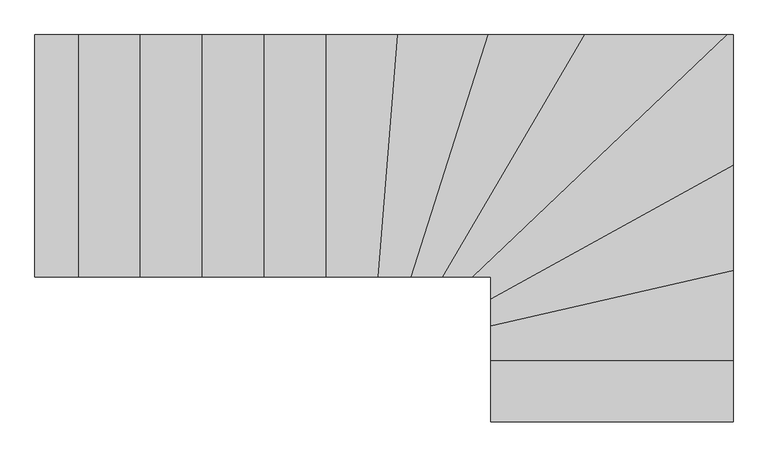
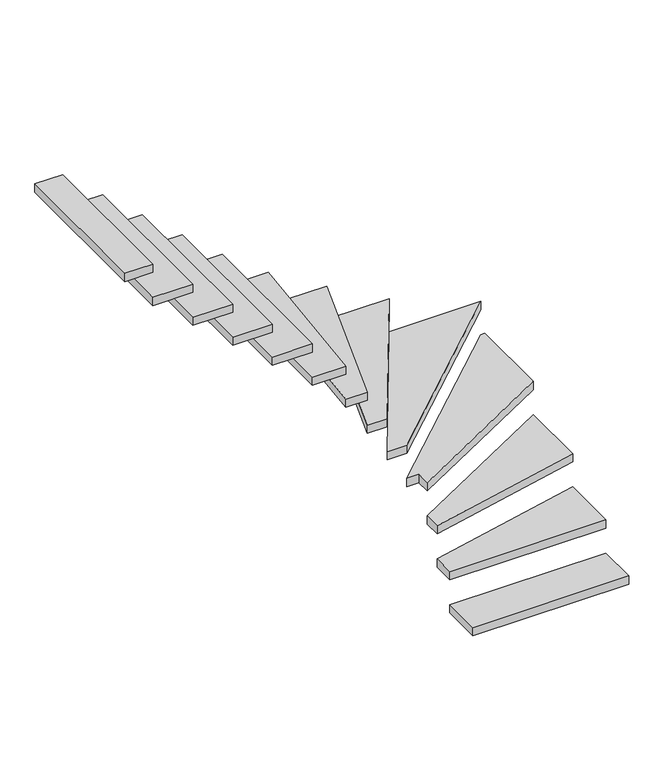
"""IFC4 building model written with IfcOpenShell, lengths in millimetres: stair geometry,   151686 :   151686."""

import ifcopenshell
import ifcopenshell.guid

model = None  # the IFC model being written
_history = None  # IfcOwnerHistory: only IFC2X3 demands one
_inside = {}  # id of a spatial element -> (the spatial element, [elements in it])
_under = {}  # id of a project, library or spatial element -> (it, [spatial elements below it])
_declared = {}  # id of a project -> (the project, [libraries it declares])
_typed = {}  # id of a type object -> (the type object, [elements of that type])
_made_of = {}  # id of a material, layer set ... -> (it, [elements and type objects made of it])


def new_model(schema):
    """Start an empty IFC model of exactly this schema.

    Asked for "IFC4X3", IfcOpenShell would pick the latest addendum, in which some entities
    have other attributes; the version numbers below select the first issue.
    IFC2X3 requires an IfcOwnerHistory on every rooted entity: one is made here for all.
    """
    global model, _history
    if schema == "IFC4X3":
        model = ifcopenshell.file(schema_version=(4, 3, 0, 0))
    else:
        model = ifcopenshell.file(schema=schema)
    _inside.clear()
    _under.clear()
    _declared.clear()
    _typed.clear()
    _made_of.clear()
    _history = None
    if model.schema == "IFC2X3":
        org = make("IfcOrganization", Name="unknown")
        user = make(
            "IfcPersonAndOrganization",
            ThePerson=make("IfcPerson", FamilyName="unknown"),
            TheOrganization=org,
        )
        app = make(
            "IfcApplication",
            ApplicationDeveloper=org,
            Version="unknown",
            ApplicationFullName="unknown",
            ApplicationIdentifier="unknown",
        )
        _history = make(
            "IfcOwnerHistory",
            OwningUser=user,
            OwningApplication=app,
            ChangeAction="ADDED",
            CreationDate=0,
        )
    return model


def make(cls, **values):
    """One entity of the class cls with the attributes given. An attribute that is None is left unset."""
    return model.create_entity(
        cls, **{name: value for name, value in values.items() if value is not None}
    )


def rooted(cls, **values):
    """An entity with a GlobalId (a new one), such as an element, a storey or a relation."""
    return make(cls, GlobalId=ifcopenshell.guid.new(), OwnerHistory=_history, **values)


def si_unit(unit_type, name, prefix=None):
    """IfcSIUnit, for example si_unit("LENGTHUNIT", "METRE", prefix="MILLI")."""
    return make("IfcSIUnit", UnitType=unit_type, Prefix=prefix, Name=name)


def assignment(units):
    """IfcUnitAssignment: the units of a project."""
    return None if units is None else make("IfcUnitAssignment", Units=units)


def point(xyz):
    """IfcCartesianPoint."""
    return None if xyz is None else make("IfcCartesianPoint", Coordinates=xyz)


def direction(xyz):
    """IfcDirection."""
    return None if xyz is None else make("IfcDirection", DirectionRatios=xyz)


def frame(location, z_axis=None, x_axis=None):
    """IfcAxis2Placement3D, a coordinate frame: its origin and axes. An axis left out is left unset."""
    return make(
        "IfcAxis2Placement3D",
        Location=point(location),
        Axis=direction(z_axis),
        RefDirection=direction(x_axis),
    )


def origin():
    """The frame at (0, 0, 0) with its axes left unset."""
    return frame((0.0, 0.0, 0.0))


def place(relative_to, where):
    """IfcLocalPlacement: puts the frame where relative to a parent placement (None: the world)."""
    return make(
        "IfcLocalPlacement", PlacementRelTo=relative_to, RelativePlacement=where
    )


def context(
    kind, dimensions, precision=None, world=None, true_north=None, identifier=None
):
    """IfcGeometricRepresentationContext, for example the 3D "Model" context."""
    return make(
        "IfcGeometricRepresentationContext",
        ContextIdentifier=identifier,
        ContextType=kind,
        CoordinateSpaceDimension=dimensions,
        Precision=precision,
        WorldCoordinateSystem=world,
        TrueNorth=true_north,
    )


def project(units=None, contexts=None):
    """IfcProject with its units and contexts."""
    return rooted(
        "IfcProject",
        Name="project",
        RepresentationContexts=contexts,
        UnitsInContext=assignment(units),
    )


def spatial(cls, under=None, at=None, **own):
    """A site, building, storey or space (cls), placed at a placement, below another one or the project."""
    s = rooted(cls, ObjectPlacement=at, **own)
    if under is not None:
        _under.setdefault(under.id(), (under, []))[1].append(s)
    return s


def polyline(points):
    """IfcPolyline through the points."""
    return make("IfcPolyline", Points=[point(p) for p in points])


def outline(outer, holes=None, kind="AREA"):
    """IfcArbitraryClosedProfileDef: a profile drawn as a closed curve; with holes, ...WithVoids."""
    if holes is None:
        return make("IfcArbitraryClosedProfileDef", ProfileType=kind, OuterCurve=outer)
    return make(
        "IfcArbitraryProfileDefWithVoids",
        ProfileType=kind,
        OuterCurve=outer,
        InnerCurves=holes,
    )


def extrude(swept, where, along, depth):
    """IfcExtrudedAreaSolid: the profile swept, set in the frame where, extruded along a direction by depth."""
    return make(
        "IfcExtrudedAreaSolid",
        SweptArea=swept,
        Position=where,
        ExtrudedDirection=direction(along),
        Depth=depth,
    )


def shape(context_of_items, identifier, shape_type, items):
    """IfcShapeRepresentation: the items that make up one representation, for example the "Body"."""
    return make(
        "IfcShapeRepresentation",
        ContextOfItems=context_of_items,
        RepresentationIdentifier=identifier,
        RepresentationType=shape_type,
        Items=items,
    )


def source(mapping_origin, context_of_items, identifier, shape_type, items):
    """IfcRepresentationMap: a shape defined once, which mapped items show again and again."""
    return make(
        "IfcRepresentationMap",
        MappingOrigin=mapping_origin,
        MappedRepresentation=shape(context_of_items, identifier, shape_type, items),
    )


def transform(
    local_origin,
    x_axis=None,
    y_axis=None,
    z_axis=None,
    scale=None,
    scale2=None,
    scale3=None,
    uniform=True,
):
    """IfcCartesianTransformationOperator3D, or its non-uniform kind. x_axis, y_axis, z_axis: its Axis1, 2, 3."""
    if uniform:
        return make(
            "IfcCartesianTransformationOperator3D",
            Axis1=direction(x_axis),
            Axis2=direction(y_axis),
            LocalOrigin=point(local_origin),
            Scale=scale,
            Axis3=direction(z_axis),
        )
    return make(
        "IfcCartesianTransformationOperator3DnonUniform",
        Axis1=direction(x_axis),
        Axis2=direction(y_axis),
        LocalOrigin=point(local_origin),
        Scale=scale,
        Axis3=direction(z_axis),
        Scale2=scale2,
        Scale3=scale3,
    )


def mapped(mapping_source, mapping_target):
    """IfcMappedItem: shows the shape of a source again, moved by a transform."""
    return make(
        "IfcMappedItem", MappingSource=mapping_source, MappingTarget=mapping_target
    )


def made_of(thing, what):
    """Note that an element or type object is made of a material, layer set ...; save() writes the relation."""
    if what is not None:
        _made_of.setdefault(what.id(), (what, []))[1].append(thing)
    return thing


def element(
    cls,
    number,
    at=None,
    inside=None,
    cuts=None,
    type_object=None,
    material=None,
    context=None,
    identifier="Body",
    shape_type=None,
    held_by="IfcProductDefinitionShape",
    body=None,
    shapes=None,
    **own,
):
    """One element of the class cls, such as IfcWall. Its Tag is "e" and its number.

    at: its placement. inside: the storey or other place that contains it. cuts: it is an
    opening in that element (IfcRelVoidsElement). A single representation is given by context,
    identifier, shape_type and body (its items); several are given by shapes. held_by: the class
    of the entity that holds the representations. save() writes the other relations.
    """
    e = rooted(cls, Tag="e%d" % number, ObjectPlacement=at, **own)
    if body is not None:
        shapes = [shape(context, identifier, shape_type, body)]
    if shapes is not None:
        e.Representation = make(held_by, Representations=shapes)
    if inside is not None:
        _inside.setdefault(inside.id(), (inside, []))[1].append(e)
    if cuts is not None:
        rooted(
            "IfcRelVoidsElement", RelatingBuildingElement=cuts, RelatedOpeningElement=e
        )
    if type_object is not None:
        _typed.setdefault(type_object.id(), (type_object, []))[1].append(e)
    return made_of(e, material)


def aggregate(whole, parts):
    """IfcRelAggregates: a whole, such as a stair, and the parts it consists of."""
    return rooted("IfcRelAggregates", RelatingObject=whole, RelatedObjects=parts)


def save(model, path):
    """Write the relations noted so far, then the file.

    IfcRelAggregates (storeys below a building ...), IfcRelContainedInSpatialStructure (elements
    in a storey), IfcRelDefinesByType, IfcRelAssociatesMaterial and IfcRelDeclares: one each for
    every whole, place, type object, material and project.
    """
    for whole, parts in _under.values():
        aggregate(whole, parts)
    for where, things in _inside.values():
        rooted(
            "IfcRelContainedInSpatialStructure",
            RelatedElements=things,
            RelatingStructure=where,
        )
    for kind, things in _typed.values():
        rooted("IfcRelDefinesByType", RelatedObjects=things, RelatingType=kind)
    for what, things in _made_of.values():
        rooted("IfcRelAssociatesMaterial", RelatedObjects=things, RelatingMaterial=what)
    for by, libraries in _declared.values():
        rooted("IfcRelDeclares", RelatingContext=by, RelatedDefinitions=libraries)
    model.write(path)


def stair_6893023c(model_context):
    return source(origin(), model_context, "Body", "SweptSolid", [
        extrude(outline(polyline([(171517.7593015, 39074.7962965), (172417.7593015, 39074.7962965), (172417.7593015, 38844.7962965), (171517.7593015, 38844.7962965), (171517.7593015, 39074.7962965)])), frame((0.0, 0.0, 3482.1428571), z_axis=(0.0, 0.0, 1.0), x_axis=(1.0, 0.0, 0.0)), (0.0, 0.0, 1.0), 50.0),
        extrude(outline(polyline([(171517.7593015, 39201.8291061), (172417.7593015, 39407.7634868), (172417.7593015, 39074.7962965), (171517.7593015, 39074.7962965), (171517.7593015, 39201.8291061)])), frame((0.0, 0.0, 3684.2857143), z_axis=(0.0, 0.0, 1.0), x_axis=(1.0, 0.0, 0.0)), (0.0, 0.0, 1.0), 50.0),
        extrude(outline(polyline([(171517.7593015, 39301.7193734), (172417.7593015, 39801.0914939), (172417.7593015, 39407.7634868), (171517.7593015, 39201.8291061), (171517.7593015, 39301.7193734)])), frame((0.0, 0.0, 3886.4285714), z_axis=(0.0, 0.0, 1.0), x_axis=(1.0, 0.0, 0.0)), (0.0, 0.0, 1.0), 50.0),
        extrude(outline(polyline([(171517.7593015, 39384.7962965), (171447.7593015, 39384.7962965), (172395.0888853, 40284.7962965), (172417.7593015, 40284.7962965), (172417.7593015, 39801.0914939), (171517.7593015, 39301.7193734), (171517.7593015, 39384.7962965)])), frame((0.0, 0.0, 4088.5714286), z_axis=(0.0, 0.0, 1.0), x_axis=(1.0, 0.0, 0.0)), (0.0, 0.0, 1.0), 50.0),
        extrude(outline(polyline([(171336.7472141, 39384.7962965), (171865.3205791, 40284.7962965), (172395.0888853, 40284.7962965), (171447.7593015, 39384.7962965), (171336.7472141, 39384.7962965)])), frame((0.0, 0.0, 4290.7142857), z_axis=(0.0, 0.0, 1.0), x_axis=(1.0, 0.0, 0.0)), (0.0, 0.0, 1.0), 50.0),
        extrude(outline(polyline([(171220.2248249, 39384.7962965), (171506.0901048, 40284.7962965), (171865.3205791, 40284.7962965), (171336.7472141, 39384.7962965), (171220.2248249, 39384.7962965)])), frame((0.0, 0.0, 4492.8571429), z_axis=(0.0, 0.0, 1.0), x_axis=(1.0, 0.0, 0.0)), (0.0, 0.0, 1.0), 50.0),
        extrude(outline(polyline([(171096.414661, 39384.7962965), (171169.9002687, 40284.7962965), (171506.0901048, 40284.7962965), (171220.2248249, 39384.7962965), (171096.414661, 39384.7962965)])), frame((0.0, 0.0, 4695.0), z_axis=(0.0, 0.0, 1.0), x_axis=(1.0, 0.0, 0.0)), (0.0, 0.0, 1.0), 50.0),
        extrude(outline(polyline([(170903.1574649, 39384.7962965), (170903.1574649, 40284.7962965), (171169.9002687, 40284.7962965), (171096.414661, 39384.7962965), (170903.1574649, 39384.7962965)])), frame((0.0, 0.0, 4897.1428571), z_axis=(0.0, 0.0, 1.0), x_axis=(1.0, 0.0, 0.0)), (0.0, 0.0, 1.0), 50.0),
        extrude(outline(polyline([(170673.1574649, 39384.7962965), (170673.1574649, 40284.7962965), (170903.1574649, 40284.7962965), (170903.1574649, 39384.7962965), (170673.1574649, 39384.7962965)])), frame((0.0, 0.0, 5099.2857143), z_axis=(0.0, 0.0, 1.0), x_axis=(1.0, 0.0, 0.0)), (0.0, 0.0, 1.0), 50.0),
        extrude(outline(polyline([(170443.1574649, 39384.7962965), (170443.1574649, 40284.7962965), (170673.1574649, 40284.7962965), (170673.1574649, 39384.7962965), (170443.1574649, 39384.7962965)])), frame((0.0, 0.0, 5301.4285714), z_axis=(0.0, 0.0, 1.0), x_axis=(1.0, 0.0, 0.0)), (0.0, 0.0, 1.0), 50.0),
        extrude(outline(polyline([(170213.1574649, 39384.7962965), (170213.1574649, 40284.7962965), (170443.1574649, 40284.7962965), (170443.1574649, 39384.7962965), (170213.1574649, 39384.7962965)])), frame((0.0, 0.0, 5503.5714286), z_axis=(0.0, 0.0, 1.0), x_axis=(1.0, 0.0, 0.0)), (0.0, 0.0, 1.0), 50.0),
        extrude(outline(polyline([(169983.1574649, 39384.7962965), (169983.1574649, 40284.7962965), (170213.1574649, 40284.7962965), (170213.1574649, 39384.7962965), (169983.1574649, 39384.7962965)])), frame((0.0, 0.0, 5705.7142857), z_axis=(0.0, 0.0, 1.0), x_axis=(1.0, 0.0, 0.0)), (0.0, 0.0, 1.0), 50.0),
        extrude(outline(polyline([(169822.7593015, 39384.7962965), (169822.7593015, 40284.7962965), (169983.1574649, 40284.7962965), (169983.1574649, 39384.7962965), (169822.7593015, 39384.7962965)])), frame((0.0, 0.0, 5907.8571429), z_axis=(0.0, 0.0, 1.0), x_axis=(1.0, 0.0, 0.0)), (0.0, 0.0, 1.0), 50.0),
    ])


if __name__ == "__main__":
    model = new_model("IFC4")
    model_context = context("Model", 3, world=origin())
    ifc_project = project(units=[si_unit("LENGTHUNIT", "METRE", prefix="MILLI")], contexts=[model_context])
    site = spatial("IfcSite", under=ifc_project)
    building = spatial("IfcBuilding", under=site)
    placement = place(None, origin())
    stair_shape = stair_6893023c(model_context)
    element("IfcStair", 1, ObjectType="  151686 :   151686", at=placement, inside=building, context=model_context, shape_type="MappedRepresentation", body=[
        mapped(stair_shape, transform((0.0, 0.0, 0.0), x_axis=(1.0, 0.0, 0.0), y_axis=(0.0, 1.0, 0.0), z_axis=(0.0, 0.0, 1.0))),
    ])
    save(model, "model.ifc")

# Revit data of these elements
# Type "  151686 :   151686"
#   Abrechnungsart = "St"
#   Allright_Bauteil_ID = "0131Tre0659044570"
#   Material = "Stahlbeton"
#   Objektname = "Treppe"
#   NameOverride = " "
#   ThermalTransmittance = 0.0000 BTU/(h·ft²·°F)
#   NosingLength = 0.000 m
#   NumberOfRiser = 14
#   NumberOfTreads = 13
#   RiserHeight = 2.021 m
#   TreadLength = 2.300 m
#   IsExternal = no
#   FireExit = no
#   HandicapAccessible = no
#   HasNonSkidSurface = no
# Element 1 (IfcStair, "  151686 :   151686")
#   Materials on its faces: "weiss"
# Materials
#   "weiss": class "Unassigned", colour RGB 255 255 255, transparency 0
